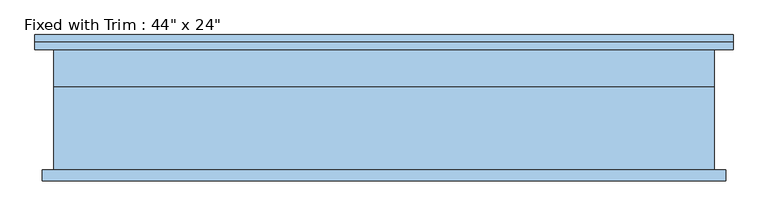
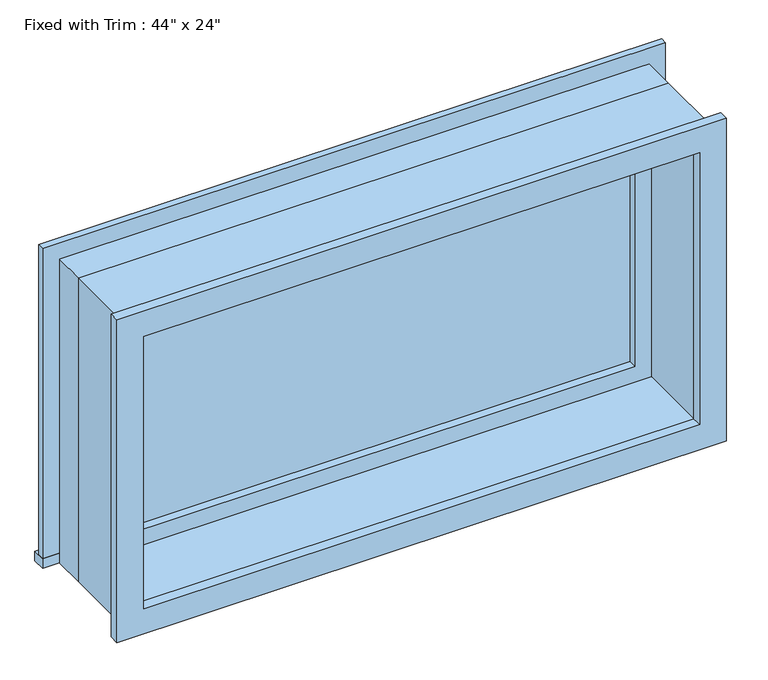
"""IFC4 building model written with IfcOpenShell, lengths in millimetres: window geometry."""

from ifc_helpers import new_model, si_unit, frame, origin, place, context, project, spatial, polyline, outline, extrude, source, transform, mapped, element, save


def window_4cd090c9(model_context):
    return source(origin(), model_context, "Body", "SweptSolid", [
        extrude(outline(polyline([(-628.65, 127.0), (552.45, 127.0), (552.45, 101.6), (-628.65, 101.6), (-628.65, 127.0)])), frame((0.0, 0.0, 914.4), z_axis=(0.0, 0.0, 1.0), x_axis=(1.0, 0.0, 0.0)), (0.0, 0.0, 1.0), 19.05),
        extrude(outline(polyline([(1504.95, -577.85), (1504.95, 501.65), (933.45, 501.65), (933.45, 552.45), (1555.75, 552.45), (1555.75, -628.65), (933.45, -628.65), (933.45, -577.85), (1504.95, -577.85)])), frame((0.0, 101.6, 0.0), z_axis=(0.0, 1.0, 0.0), x_axis=(0.0, 0.0, 1.0)), (0.0, 0.0, 1.0), 12.7),
        extrude(outline(polyline([(1543.05, 539.75), (1543.05, -615.95), (895.35, -615.95), (895.35, 539.75), (1543.05, 539.75)]), holes=[polyline([(1492.25, 488.95), (946.15, 488.95), (946.15, -565.15), (1492.25, -565.15), (1492.25, 488.95)])]), frame((0.0, -120.65, 0.0), z_axis=(0.0, 1.0, 0.0), x_axis=(0.0, 0.0, 1.0)), (0.0, 0.0, 1.0), 19.05),
        extrude(outline(polyline([(457.2, 53.975), (-533.4, 53.975), (-533.4, 66.675), (457.2, 66.675), (457.2, 53.975)])), frame((0.0, 0.0, 977.9), z_axis=(0.0, 0.0, 1.0), x_axis=(1.0, 0.0, 0.0)), (0.0, 0.0, 1.0), 482.6),
        extrude(outline(polyline([(1504.95, -577.85), (933.45, -577.85), (933.45, 501.65), (1504.95, 501.65), (1504.95, -577.85)]), holes=[polyline([(1460.5, -533.4), (1460.5, 457.2), (977.9, 457.2), (977.9, -533.4), (1460.5, -533.4)])]), frame((0.0, 38.1, 0.0), z_axis=(0.0, 1.0, 0.0), x_axis=(0.0, 0.0, 1.0)), (0.0, 0.0, 1.0), 44.45),
        extrude(outline(polyline([(1524.0, -596.9), (914.4, -596.9), (914.4, 520.7), (1524.0, 520.7), (1524.0, -596.9)]), holes=[polyline([(1492.25, -565.15), (1492.25, 488.95), (946.15, 488.95), (946.15, -565.15), (1492.25, -565.15)])]), frame((0.0, -101.6, 0.0), z_axis=(0.0, 1.0, 0.0), x_axis=(0.0, 0.0, 1.0)), (0.0, 0.0, 1.0), 139.7),
        extrude(outline(polyline([(1524.0, 520.7), (1524.0, -596.9), (914.4, -596.9), (914.4, 520.7), (1524.0, 520.7)]), holes=[polyline([(1504.95, 501.65), (933.45, 501.65), (933.45, -577.85), (1504.95, -577.85), (1504.95, 501.65)])]), frame((0.0, 38.1, 0.0), z_axis=(0.0, 1.0, 0.0), x_axis=(0.0, 0.0, 1.0)), (0.0, 0.0, 1.0), 63.5),
    ])


if __name__ == "__main__":
    model = new_model("IFC4")
    model_context = context("Model", 3, world=origin())
    ifc_project = project(units=[si_unit("LENGTHUNIT", "METRE", prefix="MILLI")], contexts=[model_context])
    site = spatial("IfcSite", under=ifc_project)
    building = spatial("IfcBuilding", under=site)
    placement = place(None, origin())
    window_shape = window_4cd090c9(model_context)
    element("IfcWindow", 1, ObjectType="Fixed with Trim : 44\" x 24\"", at=placement, inside=building, context=model_context, shape_type="MappedRepresentation", body=[
        mapped(window_shape, transform((0.0, 0.0, 0.0), x_axis=(1.0, 0.0, 0.0), y_axis=(0.0, 1.0, 0.0), z_axis=(0.0, 0.0, 1.0))),
    ])
    save(model, "model.ifc")

# Revit data of these elements
# Type "Fixed with Trim : 44\" x 24\""
#   Type Mark = "88"
#   Assembly Code = "B2020100"
#   Height = 2' - 0"
#   Default Sill Height = 3' - 0"
#   Trim Projection - Ext. = 0' - 0 1/2"
#   Trim Projection - Int. = 0' - 0 3/4"
#   Trim Width - Exterior = 0' - 2"
#   Trim Width - Interior = 0' - 2"
#   Width = 3' - 8"
#   Window Inset = 0' - 0 3/4"
#   Glass Pane Material = Glass
#   Sash Material = Sash
#   Trim Exterior Material = Trim
#   Trim Interior Material = Trim
#   Wall Closure = (empty or 0)
# Element 1 (IfcWindow, "Fixed with Trim : 44\" x 24\"")
#   Materials on its faces: "Sash", "Trim", "Glass"
# Materials
#   "Glass": class "Glass", colour RGB 0 128 192, transparency 0.75
#   "Sash": class "Wood", colour RGB 224 178 126, transparency 0
#   "Trim": class "Wood", colour RGB 224 178 126, transparency 0
